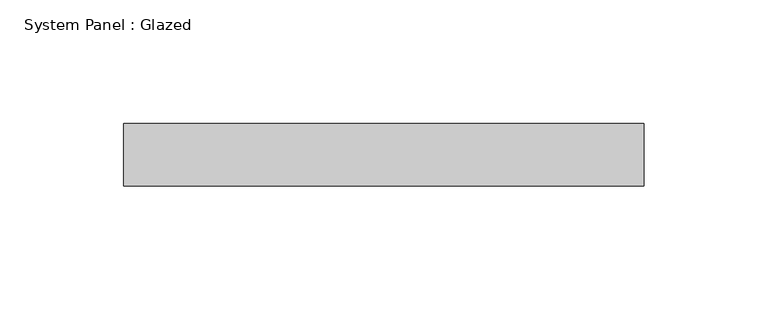
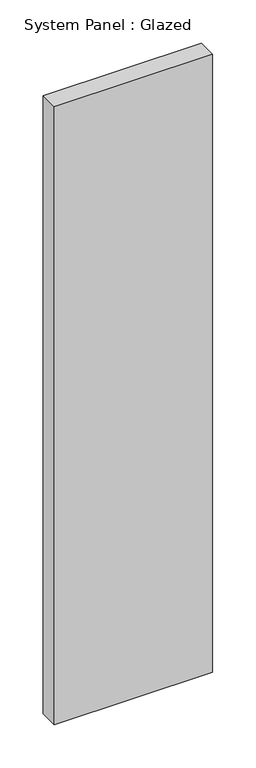
"""IFC4 building model written with IfcOpenShell, lengths in millimetres: plate geometry, System Panel : Glazed."""

from ifc_helpers import new_model, si_unit, origin, origin_with_axes, place, context, project, spatial, polyline, outline, extrude, source, transform, mapped, element, save


def system_panel_glazed_06645575(model_context):
    return source(origin(), model_context, "Body", "SweptSolid", [
        extrude(outline(polyline([(105.4575643, 19.05), (-105.4575643, 19.05), (-105.4575643, 44.45), (105.4575643, 44.45), (105.4575643, 19.05)])), origin_with_axes(), (0.0, 0.0, 1.0), 869.95),
    ])


if __name__ == "__main__":
    model = new_model("IFC4")
    model_context = context("Model", 3, world=origin())
    ifc_project = project(units=[si_unit("LENGTHUNIT", "METRE", prefix="MILLI")], contexts=[model_context])
    site = spatial("IfcSite", under=ifc_project)
    building = spatial("IfcBuilding", under=site)
    placement = place(None, origin())
    system_panel_glazed_shape = system_panel_glazed_06645575(model_context)
    element("IfcPlate", 1, ObjectType="System Panel : Glazed", at=placement, inside=building, context=model_context, shape_type="MappedRepresentation", body=[
        mapped(system_panel_glazed_shape, transform((0.0, 0.0, 0.0), x_axis=(1.0, 0.0, 0.0), y_axis=(0.0, 1.0, 0.0), z_axis=(0.0, 0.0, 1.0))),
    ])
    save(model, "model.ifc")

# Revit data of these elements
# Element 1 (IfcPlate, "System Panel : Glazed")
#   Materials on its faces: "Glass"
# Materials
#   "Glass": class "Glass", colour RGB 0 128 192, transparency 0.75
